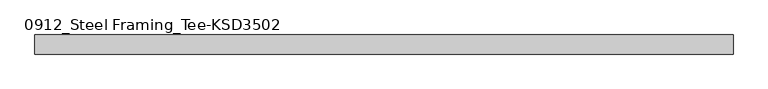
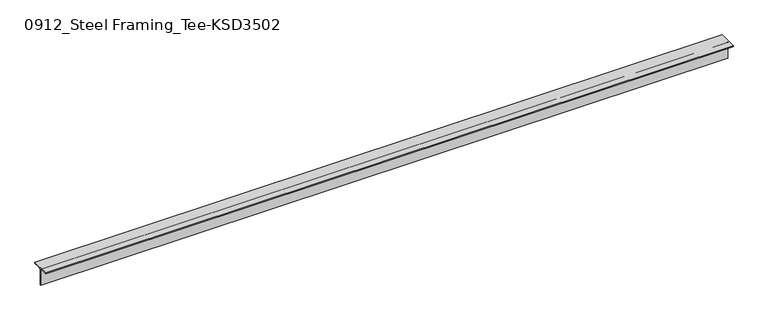
"""IFC4 building model written with IfcOpenShell, lengths in millimetres: member geometry, 0912_Steel Framing_Tee-KSD3502 : H_SB_ASB_CT-150x150x6.5x9."""

from ifc_helpers import new_model, si_unit, point, frame, frame_2d, origin, place, context, project, spatial, polyline, circle_curve, trimmed, segment, composite_curve, outline, extrude, source, transform, mapped, element, save


def member_0912_steel_framing_tee_ksd3502_64bffc7a(model_context):
    return source(origin(), model_context, "Body", "SweptSolid", [
        extrude(outline(composite_curve([segment(polyline([(-75.0, 75.0), (75.0, 75.0), (75.0, 66.0), (16.25, 66.0)]), True, "CONTINUOUS"), segment(trimmed(circle_curve(frame_2d((16.25, 53.0)), 13.0), [point((16.25, 66.0))], [point((3.25, 53.0))], True, "CARTESIAN"), True, "CONTINUOUS"), segment(polyline([(3.25, 53.0), (3.25, -75.0), (-3.25, -75.0), (-3.25, 53.0)]), True, "CONTINUOUS"), segment(trimmed(circle_curve(frame_2d((-16.25, 53.0)), 13.0), [point((-3.25, 53.0))], [point((-16.25, 66.0))], True, "CARTESIAN"), True, "CONTINUOUS"), segment(polyline([(-16.25, 66.0), (-75.0, 66.0), (-75.0, 75.0)]), True, "CONTINUOUS")], self_intersect=False)), frame((-2743.0, 0.0, 0.0), z_axis=(1.0, 0.0, 0.0), x_axis=(0.0, 1.0, 0.0)), (0.0, 0.0, 1.0), 5479.0),
    ])


if __name__ == "__main__":
    model = new_model("IFC4")
    model_context = context("Model", 3, world=origin())
    ifc_project = project(units=[si_unit("LENGTHUNIT", "METRE", prefix="MILLI")], contexts=[model_context])
    site = spatial("IfcSite", under=ifc_project)
    building = spatial("IfcBuilding", under=site)
    placement = place(None, origin())
    member_0912_steel_framing_tee_ksd3502_shape = member_0912_steel_framing_tee_ksd3502_64bffc7a(model_context)
    element("IfcMember", 1, ObjectType="0912_Steel Framing_Tee-KSD3502 : H_SB_ASB_CT-150x150x6.5x9", at=placement, inside=building, context=model_context, shape_type="MappedRepresentation", body=[
        mapped(member_0912_steel_framing_tee_ksd3502_shape, transform((0.0, 0.0, 0.0), x_axis=(1.0, 0.0, 0.0), y_axis=(0.0, 1.0, 0.0), z_axis=(0.0, 0.0, 1.0))),
    ])
    save(model, "model.ifc")

# Revit data of these elements
# Type "0912_Steel Framing_Tee-KSD3502 : H_SB_ASB_CT-150x150x6.5x9"
#   H_WM Code_1 = "S01AA003-00001 | Main Steel Structure Fabrication Work | Shelter/Building | Light Steel - Standard (30KG/M>Weight) | Material: (   )"
#   H_WM Code_2 = "S03AA029-00001 | Main Steel Structure Erection Work | Shelter/Building | Light Steel (30KG/M>Weight) | Material: (   )"
#   H_WM Code_3 = "S01AA010-00001 | Main Steel Structure Fabrication Work | Shelter/Building | Steel Painting/Coating | for Non-Fireproofed Steel Surface, Surface Preparation, Primer, Second & Final Coat | Material: (   )"
#   H_Q'ty Cal Type Tag = "SB-Q2"
#   Width = 15.0 cm
#   Web Thickness = 0.65 cm
#   Web Fillet = 1.3 cm
#   Section Area = 23.39 cm²
#   Perimeter = 0.60 m²/m
#   Nominal Weight = 18.40 kgf/m
#   Height = 15.0 cm
#   Flange Thickness = 0.9 cm
#   Centroid Vertical = 7.5 cm
#   Centroid Horizontal = 7.5 cm
#   Length [instance default] = 1.5000 m
#   Structural Material [instance default] = Steel, 45-345
#   Warping Constant = (empty or 0)
#   Torsional Moment of Inertia = 0
#   Section Name Key = ""
#   Plastic Modulus weak axis = 0
#   Plastic Modulus strong axis = 0
#   Moment of Inertia weak axis = 0
#   Moment of Inertia strong axis = 0
#   Elastic Modulus weak axis = 0
#   Elastic Modulus strong axis = 0
#   Bolt Spacing = 0
#   Assembly Code = ""
# Element 1 (IfcMember, "0912_Steel Framing_Tee-KSD3502 : H_SB_ASB_CT-150x150x6.5x9")
#   Structural Material = none
# Materials
#   "Steel, 45-345": class "Metal", colour RGB 189 187 185, transparency 0, Description = "Steel 345 MPa", Cost = 0
